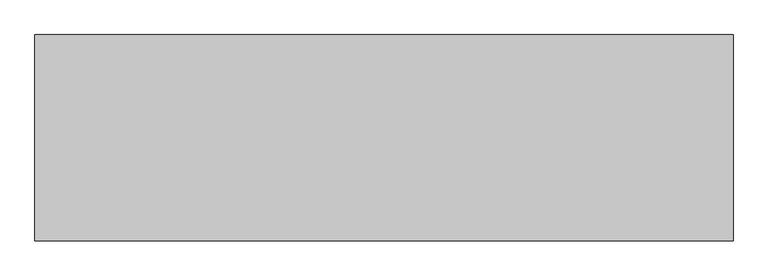
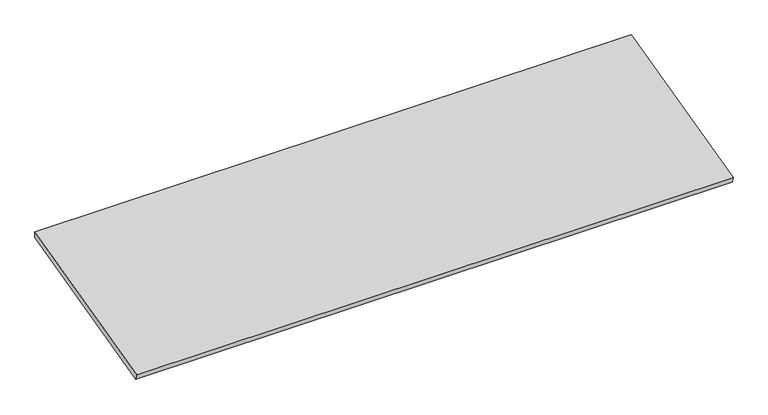
"""IFC4 building model written with IfcOpenShell, lengths in millimetres: proxy geometry, Plywood009 3213 : Plywood009 3213."""

from ifc_helpers import new_model, si_unit, frame, origin, place, context, project, spatial, polyline, outline, extrude, source, transform, mapped, element, save


def generic_models_a679d8c2(model_context):
    return source(origin(), model_context, "Body", "SweptSolid", [
        extrude(outline(polyline([(10765.3875834, 43886.744178), (10765.3875834, 43867.1075714), (10179.0930265, 43720.5356366), (10174.4726032, 43739.01733), (10765.3875834, 43886.744178)])), frame((3694.0383192, 0.0, 0.0), z_axis=(1.0, 0.0, 0.0), x_axis=(0.0, 1.0, 0.0)), (0.0, 0.0, 1.0), 2000.25),
    ])


if __name__ == "__main__":
    model = new_model("IFC4")
    model_context = context("Model", 3, world=origin())
    ifc_project = project(units=[si_unit("LENGTHUNIT", "METRE", prefix="MILLI")], contexts=[model_context])
    site = spatial("IfcSite", under=ifc_project)
    building = spatial("IfcBuilding", under=site)
    placement = place(None, origin())
    generic_models_shape = generic_models_a679d8c2(model_context)
    element("IfcBuildingElementProxy", 1, Name="Plywood009 3213 : Plywood009 3213", ObjectType="Plywood009 3213 : Plywood009 3213", at=placement, inside=building, context=model_context, shape_type="MappedRepresentation", body=[
        mapped(generic_models_shape, transform((0.0, 0.0, 0.0), x_axis=(1.0, 0.0, 0.0), y_axis=(0.0, 1.0, 0.0), z_axis=(0.0, 0.0, 1.0))),
    ])
    save(model, "model.ifc")

# Revit data of these elements
# Type "Plywood009 3213 : Plywood009 3213"
#   NameOverride = "Plywood009"
# Element 1 (IfcBuildingElementProxy, "Plywood009 3213 : Plywood009 3213")
#   Materials on its faces: "CDX PLYWOOD - SEE STRUCTURAL DWGS"
# Materials
#   "CDX PLYWOOD - SEE STRUCTURAL DWGS": class "Unassigned", colour RGB 177 130 114, transparency 0, Cost = 0
